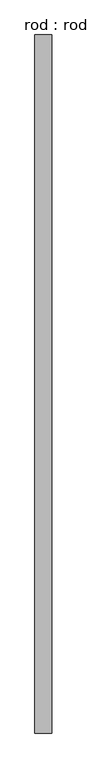
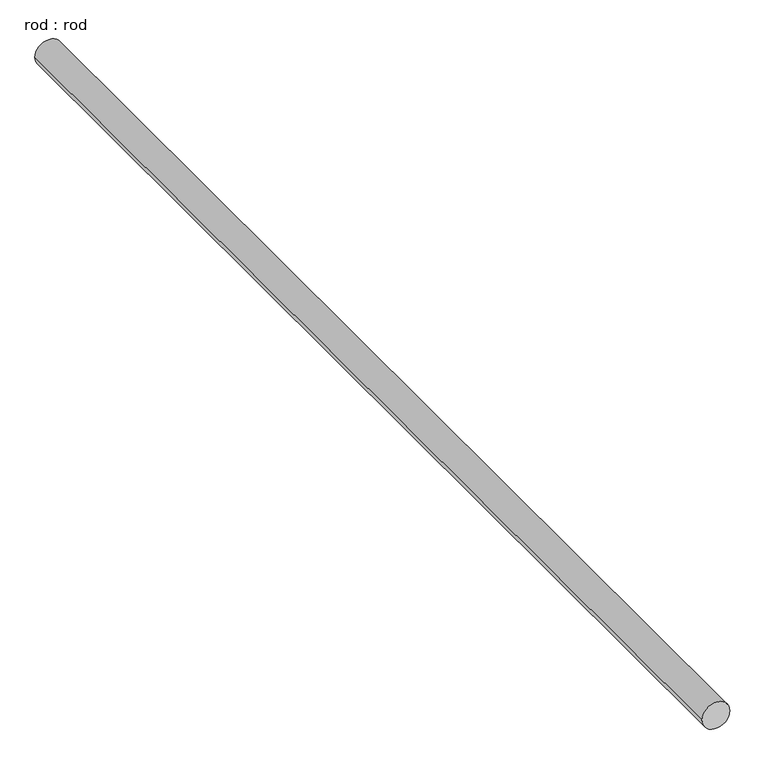
"""IFC4 building model written with IfcOpenShell, lengths in millimetres: proxy geometry, rod : rod."""

from ifc_helpers import new_model, si_unit, point, frame, frame_2d, origin, place, context, project, spatial, circle_curve, trimmed, segment, composite_curve, outline, extrude, source, transform, mapped, element, save


def rod_rod_e8285aa7(model_context):
    return source(origin(), model_context, "Body", "SweptSolid", [
        extrude(outline(composite_curve([segment(trimmed(circle_curve(frame_2d((0.0108462, 0.0)), 200.0), [point((0.0108462, 200.0))], [point((0.0108462, -200.0))], False, "CARTESIAN"), True, "CONTINUOUS"), segment(trimmed(circle_curve(frame_2d((0.0108462, 0.0)), 200.0), [point((0.0108462, -200.0))], [point((0.0108462, 200.0))], False, "CARTESIAN"), True, "CONTINUOUS")], self_intersect=False)), frame((0.0, -4216.4189579, 0.0), z_axis=(0.0, 1.0, 0.0), x_axis=(0.0, 0.0, 1.0)), (0.0, 0.0, 1.0), 16618.2951465),
    ])


if __name__ == "__main__":
    model = new_model("IFC4")
    model_context = context("Model", 3, world=origin())
    ifc_project = project(units=[si_unit("LENGTHUNIT", "METRE", prefix="MILLI")], contexts=[model_context])
    site = spatial("IfcSite", under=ifc_project)
    building = spatial("IfcBuilding", under=site)
    placement = place(None, origin())
    rod_rod_shape = rod_rod_e8285aa7(model_context)
    element("IfcBuildingElementProxy", 1, Name="rod : rod", ObjectType="rod : rod", at=placement, inside=building, context=model_context, shape_type="MappedRepresentation", body=[
        mapped(rod_rod_shape, transform((0.0, 0.0, 0.0), x_axis=(1.0, 0.0, 0.0), y_axis=(0.0, 1.0, 0.0), z_axis=(0.0, 0.0, 1.0))),
    ])
    save(model, "model.ifc")

# Revit data of these elements
# Type "rod : rod"
#   Default Elevation = 0
